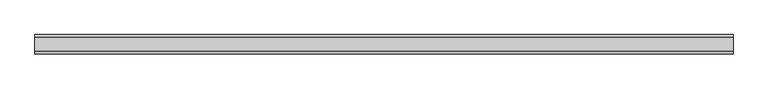
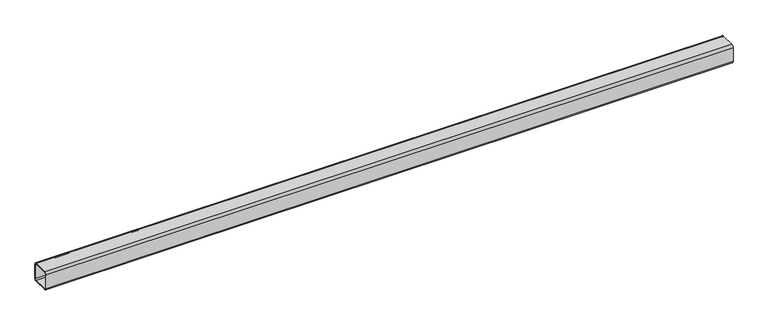
"""IFC4 building model written with IfcOpenShell, lengths in millimetres: beam geometry, Гнутый прямоугольный профиль (Трубы 30245-94) Балки : гнутый прямоуг. проф. 100x6."""

import ifcopenshell
import ifcopenshell.guid

model = None  # the IFC model being written
_history = None  # IfcOwnerHistory: only IFC2X3 demands one
_inside = {}  # id of a spatial element -> (the spatial element, [elements in it])
_under = {}  # id of a project, library or spatial element -> (it, [spatial elements below it])
_declared = {}  # id of a project -> (the project, [libraries it declares])
_typed = {}  # id of a type object -> (the type object, [elements of that type])
_made_of = {}  # id of a material, layer set ... -> (it, [elements and type objects made of it])


def new_model(schema):
    """Start an empty IFC model of exactly this schema.

    Asked for "IFC4X3", IfcOpenShell would pick the latest addendum, in which some entities
    have other attributes; the version numbers below select the first issue.
    IFC2X3 requires an IfcOwnerHistory on every rooted entity: one is made here for all.
    """
    global model, _history
    if schema == "IFC4X3":
        model = ifcopenshell.file(schema_version=(4, 3, 0, 0))
    else:
        model = ifcopenshell.file(schema=schema)
    _inside.clear()
    _under.clear()
    _declared.clear()
    _typed.clear()
    _made_of.clear()
    _history = None
    if model.schema == "IFC2X3":
        org = make("IfcOrganization", Name="unknown")
        user = make(
            "IfcPersonAndOrganization",
            ThePerson=make("IfcPerson", FamilyName="unknown"),
            TheOrganization=org,
        )
        app = make(
            "IfcApplication",
            ApplicationDeveloper=org,
            Version="unknown",
            ApplicationFullName="unknown",
            ApplicationIdentifier="unknown",
        )
        _history = make(
            "IfcOwnerHistory",
            OwningUser=user,
            OwningApplication=app,
            ChangeAction="ADDED",
            CreationDate=0,
        )
    return model


def make(cls, **values):
    """One entity of the class cls with the attributes given. An attribute that is None is left unset."""
    return model.create_entity(
        cls, **{name: value for name, value in values.items() if value is not None}
    )


def rooted(cls, **values):
    """An entity with a GlobalId (a new one), such as an element, a storey or a relation."""
    return make(cls, GlobalId=ifcopenshell.guid.new(), OwnerHistory=_history, **values)


def si_unit(unit_type, name, prefix=None):
    """IfcSIUnit, for example si_unit("LENGTHUNIT", "METRE", prefix="MILLI")."""
    return make("IfcSIUnit", UnitType=unit_type, Prefix=prefix, Name=name)


def assignment(units):
    """IfcUnitAssignment: the units of a project."""
    return None if units is None else make("IfcUnitAssignment", Units=units)


def point(xyz):
    """IfcCartesianPoint."""
    return None if xyz is None else make("IfcCartesianPoint", Coordinates=xyz)


def direction(xyz):
    """IfcDirection."""
    return None if xyz is None else make("IfcDirection", DirectionRatios=xyz)


def frame(location, z_axis=None, x_axis=None):
    """IfcAxis2Placement3D, a coordinate frame: its origin and axes. An axis left out is left unset."""
    return make(
        "IfcAxis2Placement3D",
        Location=point(location),
        Axis=direction(z_axis),
        RefDirection=direction(x_axis),
    )


def frame_2d(location, x_axis=None):
    """IfcAxis2Placement2D, a coordinate frame in the plane: its origin and x axis."""
    return make(
        "IfcAxis2Placement2D", Location=point(location), RefDirection=direction(x_axis)
    )


def origin():
    """The frame at (0, 0, 0) with its axes left unset."""
    return frame((0.0, 0.0, 0.0))


def place(relative_to, where):
    """IfcLocalPlacement: puts the frame where relative to a parent placement (None: the world)."""
    return make(
        "IfcLocalPlacement", PlacementRelTo=relative_to, RelativePlacement=where
    )


def context(
    kind, dimensions, precision=None, world=None, true_north=None, identifier=None
):
    """IfcGeometricRepresentationContext, for example the 3D "Model" context."""
    return make(
        "IfcGeometricRepresentationContext",
        ContextIdentifier=identifier,
        ContextType=kind,
        CoordinateSpaceDimension=dimensions,
        Precision=precision,
        WorldCoordinateSystem=world,
        TrueNorth=true_north,
    )


def project(units=None, contexts=None):
    """IfcProject with its units and contexts."""
    return rooted(
        "IfcProject",
        Name="project",
        RepresentationContexts=contexts,
        UnitsInContext=assignment(units),
    )


def spatial(cls, under=None, at=None, **own):
    """A site, building, storey or space (cls), placed at a placement, below another one or the project."""
    s = rooted(cls, ObjectPlacement=at, **own)
    if under is not None:
        _under.setdefault(under.id(), (under, []))[1].append(s)
    return s


def polyline(points):
    """IfcPolyline through the points."""
    return make("IfcPolyline", Points=[point(p) for p in points])


def circle_curve(where, radius):
    """IfcCircle in the frame where."""
    return make("IfcCircle", Position=where, Radius=radius)


def trimmed(basis, trim1, trim2, sense, master):
    """IfcTrimmedCurve: the piece of a basis curve between two trims."""
    return make(
        "IfcTrimmedCurve",
        BasisCurve=basis,
        Trim1=trim1,
        Trim2=trim2,
        SenseAgreement=sense,
        MasterRepresentation=master,
    )


def segment(curve, same_sense, transition):
    """IfcCompositeCurveSegment."""
    return make(
        "IfcCompositeCurveSegment",
        Transition=transition,
        SameSense=same_sense,
        ParentCurve=curve,
    )


def composite_curve(segments, self_intersect=None):
    """IfcCompositeCurve: segments joined end to end."""
    return make("IfcCompositeCurve", Segments=segments, SelfIntersect=self_intersect)


def outline(outer, holes=None, kind="AREA"):
    """IfcArbitraryClosedProfileDef: a profile drawn as a closed curve; with holes, ...WithVoids."""
    if holes is None:
        return make("IfcArbitraryClosedProfileDef", ProfileType=kind, OuterCurve=outer)
    return make(
        "IfcArbitraryProfileDefWithVoids",
        ProfileType=kind,
        OuterCurve=outer,
        InnerCurves=holes,
    )


def extrude(swept, where, along, depth):
    """IfcExtrudedAreaSolid: the profile swept, set in the frame where, extruded along a direction by depth."""
    return make(
        "IfcExtrudedAreaSolid",
        SweptArea=swept,
        Position=where,
        ExtrudedDirection=direction(along),
        Depth=depth,
    )


def shape(context_of_items, identifier, shape_type, items):
    """IfcShapeRepresentation: the items that make up one representation, for example the "Body"."""
    return make(
        "IfcShapeRepresentation",
        ContextOfItems=context_of_items,
        RepresentationIdentifier=identifier,
        RepresentationType=shape_type,
        Items=items,
    )


def source(mapping_origin, context_of_items, identifier, shape_type, items):
    """IfcRepresentationMap: a shape defined once, which mapped items show again and again."""
    return make(
        "IfcRepresentationMap",
        MappingOrigin=mapping_origin,
        MappedRepresentation=shape(context_of_items, identifier, shape_type, items),
    )


def transform(
    local_origin,
    x_axis=None,
    y_axis=None,
    z_axis=None,
    scale=None,
    scale2=None,
    scale3=None,
    uniform=True,
):
    """IfcCartesianTransformationOperator3D, or its non-uniform kind. x_axis, y_axis, z_axis: its Axis1, 2, 3."""
    if uniform:
        return make(
            "IfcCartesianTransformationOperator3D",
            Axis1=direction(x_axis),
            Axis2=direction(y_axis),
            LocalOrigin=point(local_origin),
            Scale=scale,
            Axis3=direction(z_axis),
        )
    return make(
        "IfcCartesianTransformationOperator3DnonUniform",
        Axis1=direction(x_axis),
        Axis2=direction(y_axis),
        LocalOrigin=point(local_origin),
        Scale=scale,
        Axis3=direction(z_axis),
        Scale2=scale2,
        Scale3=scale3,
    )


def mapped(mapping_source, mapping_target):
    """IfcMappedItem: shows the shape of a source again, moved by a transform."""
    return make(
        "IfcMappedItem", MappingSource=mapping_source, MappingTarget=mapping_target
    )


def made_of(thing, what):
    """Note that an element or type object is made of a material, layer set ...; save() writes the relation."""
    if what is not None:
        _made_of.setdefault(what.id(), (what, []))[1].append(thing)
    return thing


def element(
    cls,
    number,
    at=None,
    inside=None,
    cuts=None,
    type_object=None,
    material=None,
    context=None,
    identifier="Body",
    shape_type=None,
    held_by="IfcProductDefinitionShape",
    body=None,
    shapes=None,
    **own,
):
    """One element of the class cls, such as IfcWall. Its Tag is "e" and its number.

    at: its placement. inside: the storey or other place that contains it. cuts: it is an
    opening in that element (IfcRelVoidsElement). A single representation is given by context,
    identifier, shape_type and body (its items); several are given by shapes. held_by: the class
    of the entity that holds the representations. save() writes the other relations.
    """
    e = rooted(cls, Tag="e%d" % number, ObjectPlacement=at, **own)
    if body is not None:
        shapes = [shape(context, identifier, shape_type, body)]
    if shapes is not None:
        e.Representation = make(held_by, Representations=shapes)
    if inside is not None:
        _inside.setdefault(inside.id(), (inside, []))[1].append(e)
    if cuts is not None:
        rooted(
            "IfcRelVoidsElement", RelatingBuildingElement=cuts, RelatedOpeningElement=e
        )
    if type_object is not None:
        _typed.setdefault(type_object.id(), (type_object, []))[1].append(e)
    return made_of(e, material)


def aggregate(whole, parts):
    """IfcRelAggregates: a whole, such as a stair, and the parts it consists of."""
    return rooted("IfcRelAggregates", RelatingObject=whole, RelatedObjects=parts)


def save(model, path):
    """Write the relations noted so far, then the file.

    IfcRelAggregates (storeys below a building ...), IfcRelContainedInSpatialStructure (elements
    in a storey), IfcRelDefinesByType, IfcRelAssociatesMaterial and IfcRelDeclares: one each for
    every whole, place, type object, material and project.
    """
    for whole, parts in _under.values():
        aggregate(whole, parts)
    for where, things in _inside.values():
        rooted(
            "IfcRelContainedInSpatialStructure",
            RelatedElements=things,
            RelatingStructure=where,
        )
    for kind, things in _typed.values():
        rooted("IfcRelDefinesByType", RelatedObjects=things, RelatingType=kind)
    for what, things in _made_of.values():
        rooted("IfcRelAssociatesMaterial", RelatedObjects=things, RelatingMaterial=what)
    for by, libraries in _declared.values():
        rooted("IfcRelDeclares", RelatingContext=by, RelatedDefinitions=libraries)
    model.write(path)


def beam_533c434b(model_context):
    return source(origin(), model_context, "Body", "SweptSolid", [
        extrude(outline(composite_curve([segment(polyline([(-38.0, 50.0), (38.0, 50.0)]), True, "CONTINUOUS"), segment(trimmed(circle_curve(frame_2d((38.0, 38.0)), 12.0), [point((38.0, 50.0))], [point((50.0, 38.0))], False, "CARTESIAN"), True, "CONTINUOUS"), segment(polyline([(50.0, 38.0), (50.0, -38.0)]), True, "CONTINUOUS"), segment(trimmed(circle_curve(frame_2d((38.0, -38.0)), 12.0), [point((50.0, -38.0))], [point((38.0, -50.0))], False, "CARTESIAN"), True, "CONTINUOUS"), segment(polyline([(38.0, -50.0), (-38.0, -50.0)]), True, "CONTINUOUS"), segment(trimmed(circle_curve(frame_2d((-38.0, -38.0)), 12.0), [point((-38.0, -50.0))], [point((-50.0, -38.0))], False, "CARTESIAN"), True, "CONTINUOUS"), segment(polyline([(-50.0, -38.0), (-50.0, 38.0)]), True, "CONTINUOUS"), segment(trimmed(circle_curve(frame_2d((-38.0, 38.0)), 12.0), [point((-50.0, 38.0))], [point((-38.0, 50.0))], False, "CARTESIAN"), True, "CONTINUOUS")], self_intersect=False), holes=[composite_curve([segment(trimmed(circle_curve(frame_2d((-38.0, 38.0)), 6.0), [point((-38.0, 44.0))], [point((-44.0, 38.0))], True, "CARTESIAN"), True, "CONTINUOUS"), segment(polyline([(-44.0, 38.0), (-44.0, -38.0)]), True, "CONTINUOUS"), segment(trimmed(circle_curve(frame_2d((-38.0, -38.0)), 6.0), [point((-44.0, -38.0))], [point((-38.0, -44.0))], True, "CARTESIAN"), True, "CONTINUOUS"), segment(polyline([(-38.0, -44.0), (38.0, -44.0)]), True, "CONTINUOUS"), segment(trimmed(circle_curve(frame_2d((38.0, -38.0)), 6.0), [point((38.0, -44.0))], [point((44.0, -38.0))], True, "CARTESIAN"), True, "CONTINUOUS"), segment(polyline([(44.0, -38.0), (44.0, 38.0)]), True, "CONTINUOUS"), segment(trimmed(circle_curve(frame_2d((38.0, 38.0)), 6.0), [point((44.0, 38.0))], [point((38.0, 44.0))], True, "CARTESIAN"), True, "CONTINUOUS"), segment(polyline([(38.0, 44.0), (-38.0, 44.0)]), True, "CONTINUOUS")], self_intersect=False)]), frame((-1817.0, 0.0, 0.0), z_axis=(1.0, 0.0, 0.0), x_axis=(0.0, 1.0, 0.0)), (0.0, 0.0, 1.0), 3634.0),
    ])


if __name__ == "__main__":
    model = new_model("IFC4")
    model_context = context("Model", 3, world=origin())
    ifc_project = project(units=[si_unit("LENGTHUNIT", "METRE", prefix="MILLI")], contexts=[model_context])
    site = spatial("IfcSite", under=ifc_project)
    building = spatial("IfcBuilding", under=site)
    placement = place(None, origin())
    beam_shape = beam_533c434b(model_context)
    element("IfcBeam", 1, ObjectType="Гнутый прямоугольный профиль (Трубы 30245-94) Балки : гнутый прямоуг. проф. 100x6", at=placement, inside=building, context=model_context, shape_type="MappedRepresentation", body=[
        mapped(beam_shape, transform((0.0, 0.0, 0.0), x_axis=(1.0, 0.0, 0.0), y_axis=(0.0, 1.0, 0.0), z_axis=(0.0, 0.0, 1.0))),
    ])
    save(model, "model.ifc")

# Revit data of these elements
# Type "Гнутый прямоугольный профиль (Трубы 30245-94) Балки : гнутый прямоуг. проф. 100x6"
#   ri = 12 mm
#   ra = 6 mm
#   W = 0.173578
#   Vz = 50 mm
#   Vy = 50 mm
#   Vpz = 50 mm
#   Vpy = 50 mm
#   Length [instance default] = 1500 mm
#   bf = 100 mm
#   d = 100 mm
#   tf = 6 mm
#   tw = 6 mm
#   A = 0.00226 m²
#   Structural Material [instance default] = Металл - Сталь - 345 МПa
#   Assembly Code = ""
# Element 1 (IfcBeam, "Гнутый прямоугольный профиль (Трубы 30245-94) Балки : гнутый прямоуг. проф. 100x6")
#   Structural Material = C235
#   Materials on its faces: "C235"
# Materials
#   "Металл - Сталь - 345 МПa": class "Металл", colour RGB 247 247 247, transparency 0
#   "C235": class "Не назначено", colour RGB 0 0 0, transparency 0
